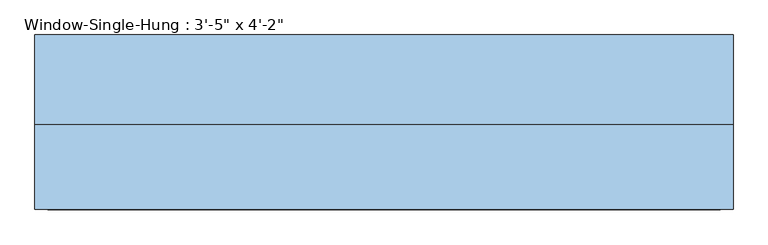
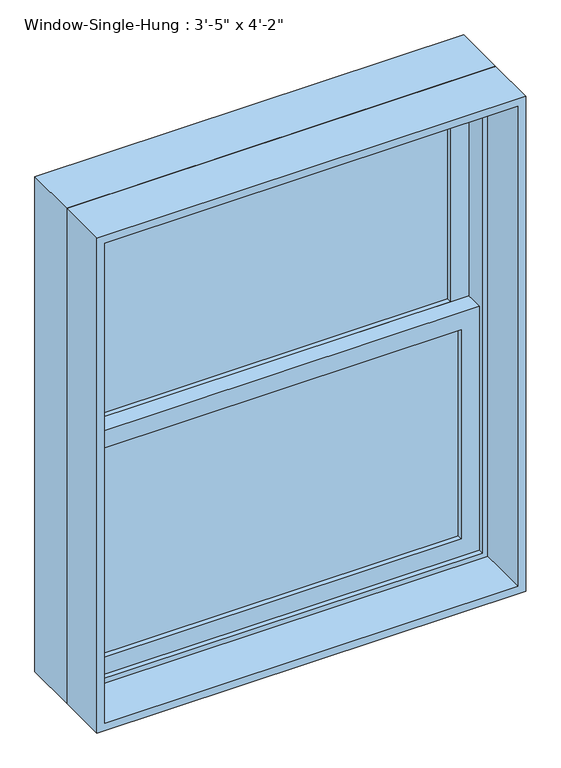
"""IFC4 building model written with IfcOpenShell, lengths in millimetres: window geometry."""

import ifcopenshell
import ifcopenshell.guid

model = None  # the IFC model being written
_history = None  # IfcOwnerHistory: only IFC2X3 demands one
_inside = {}  # id of a spatial element -> (the spatial element, [elements in it])
_under = {}  # id of a project, library or spatial element -> (it, [spatial elements below it])
_declared = {}  # id of a project -> (the project, [libraries it declares])
_typed = {}  # id of a type object -> (the type object, [elements of that type])
_made_of = {}  # id of a material, layer set ... -> (it, [elements and type objects made of it])


def new_model(schema):
    """Start an empty IFC model of exactly this schema.

    Asked for "IFC4X3", IfcOpenShell would pick the latest addendum, in which some entities
    have other attributes; the version numbers below select the first issue.
    IFC2X3 requires an IfcOwnerHistory on every rooted entity: one is made here for all.
    """
    global model, _history
    if schema == "IFC4X3":
        model = ifcopenshell.file(schema_version=(4, 3, 0, 0))
    else:
        model = ifcopenshell.file(schema=schema)
    _inside.clear()
    _under.clear()
    _declared.clear()
    _typed.clear()
    _made_of.clear()
    _history = None
    if model.schema == "IFC2X3":
        org = make("IfcOrganization", Name="unknown")
        user = make(
            "IfcPersonAndOrganization",
            ThePerson=make("IfcPerson", FamilyName="unknown"),
            TheOrganization=org,
        )
        app = make(
            "IfcApplication",
            ApplicationDeveloper=org,
            Version="unknown",
            ApplicationFullName="unknown",
            ApplicationIdentifier="unknown",
        )
        _history = make(
            "IfcOwnerHistory",
            OwningUser=user,
            OwningApplication=app,
            ChangeAction="ADDED",
            CreationDate=0,
        )
    return model


def make(cls, **values):
    """One entity of the class cls with the attributes given. An attribute that is None is left unset."""
    return model.create_entity(
        cls, **{name: value for name, value in values.items() if value is not None}
    )


def rooted(cls, **values):
    """An entity with a GlobalId (a new one), such as an element, a storey or a relation."""
    return make(cls, GlobalId=ifcopenshell.guid.new(), OwnerHistory=_history, **values)


def si_unit(unit_type, name, prefix=None):
    """IfcSIUnit, for example si_unit("LENGTHUNIT", "METRE", prefix="MILLI")."""
    return make("IfcSIUnit", UnitType=unit_type, Prefix=prefix, Name=name)


def assignment(units):
    """IfcUnitAssignment: the units of a project."""
    return None if units is None else make("IfcUnitAssignment", Units=units)


def point(xyz):
    """IfcCartesianPoint."""
    return None if xyz is None else make("IfcCartesianPoint", Coordinates=xyz)


def direction(xyz):
    """IfcDirection."""
    return None if xyz is None else make("IfcDirection", DirectionRatios=xyz)


def frame(location, z_axis=None, x_axis=None):
    """IfcAxis2Placement3D, a coordinate frame: its origin and axes. An axis left out is left unset."""
    return make(
        "IfcAxis2Placement3D",
        Location=point(location),
        Axis=direction(z_axis),
        RefDirection=direction(x_axis),
    )


def origin():
    """The frame at (0, 0, 0) with its axes left unset."""
    return frame((0.0, 0.0, 0.0))


def place(relative_to, where):
    """IfcLocalPlacement: puts the frame where relative to a parent placement (None: the world)."""
    return make(
        "IfcLocalPlacement", PlacementRelTo=relative_to, RelativePlacement=where
    )


def context(
    kind, dimensions, precision=None, world=None, true_north=None, identifier=None
):
    """IfcGeometricRepresentationContext, for example the 3D "Model" context."""
    return make(
        "IfcGeometricRepresentationContext",
        ContextIdentifier=identifier,
        ContextType=kind,
        CoordinateSpaceDimension=dimensions,
        Precision=precision,
        WorldCoordinateSystem=world,
        TrueNorth=true_north,
    )


def project(units=None, contexts=None):
    """IfcProject with its units and contexts."""
    return rooted(
        "IfcProject",
        Name="project",
        RepresentationContexts=contexts,
        UnitsInContext=assignment(units),
    )


def spatial(cls, under=None, at=None, **own):
    """A site, building, storey or space (cls), placed at a placement, below another one or the project."""
    s = rooted(cls, ObjectPlacement=at, **own)
    if under is not None:
        _under.setdefault(under.id(), (under, []))[1].append(s)
    return s


def polyline(points):
    """IfcPolyline through the points."""
    return make("IfcPolyline", Points=[point(p) for p in points])


def outline(outer, holes=None, kind="AREA"):
    """IfcArbitraryClosedProfileDef: a profile drawn as a closed curve; with holes, ...WithVoids."""
    if holes is None:
        return make("IfcArbitraryClosedProfileDef", ProfileType=kind, OuterCurve=outer)
    return make(
        "IfcArbitraryProfileDefWithVoids",
        ProfileType=kind,
        OuterCurve=outer,
        InnerCurves=holes,
    )


def extrude(swept, where, along, depth):
    """IfcExtrudedAreaSolid: the profile swept, set in the frame where, extruded along a direction by depth."""
    return make(
        "IfcExtrudedAreaSolid",
        SweptArea=swept,
        Position=where,
        ExtrudedDirection=direction(along),
        Depth=depth,
    )


def shape(context_of_items, identifier, shape_type, items):
    """IfcShapeRepresentation: the items that make up one representation, for example the "Body"."""
    return make(
        "IfcShapeRepresentation",
        ContextOfItems=context_of_items,
        RepresentationIdentifier=identifier,
        RepresentationType=shape_type,
        Items=items,
    )


def source(mapping_origin, context_of_items, identifier, shape_type, items):
    """IfcRepresentationMap: a shape defined once, which mapped items show again and again."""
    return make(
        "IfcRepresentationMap",
        MappingOrigin=mapping_origin,
        MappedRepresentation=shape(context_of_items, identifier, shape_type, items),
    )


def transform(
    local_origin,
    x_axis=None,
    y_axis=None,
    z_axis=None,
    scale=None,
    scale2=None,
    scale3=None,
    uniform=True,
):
    """IfcCartesianTransformationOperator3D, or its non-uniform kind. x_axis, y_axis, z_axis: its Axis1, 2, 3."""
    if uniform:
        return make(
            "IfcCartesianTransformationOperator3D",
            Axis1=direction(x_axis),
            Axis2=direction(y_axis),
            LocalOrigin=point(local_origin),
            Scale=scale,
            Axis3=direction(z_axis),
        )
    return make(
        "IfcCartesianTransformationOperator3DnonUniform",
        Axis1=direction(x_axis),
        Axis2=direction(y_axis),
        LocalOrigin=point(local_origin),
        Scale=scale,
        Axis3=direction(z_axis),
        Scale2=scale2,
        Scale3=scale3,
    )


def mapped(mapping_source, mapping_target):
    """IfcMappedItem: shows the shape of a source again, moved by a transform."""
    return make(
        "IfcMappedItem", MappingSource=mapping_source, MappingTarget=mapping_target
    )


def made_of(thing, what):
    """Note that an element or type object is made of a material, layer set ...; save() writes the relation."""
    if what is not None:
        _made_of.setdefault(what.id(), (what, []))[1].append(thing)
    return thing


def element(
    cls,
    number,
    at=None,
    inside=None,
    cuts=None,
    type_object=None,
    material=None,
    context=None,
    identifier="Body",
    shape_type=None,
    held_by="IfcProductDefinitionShape",
    body=None,
    shapes=None,
    **own,
):
    """One element of the class cls, such as IfcWall. Its Tag is "e" and its number.

    at: its placement. inside: the storey or other place that contains it. cuts: it is an
    opening in that element (IfcRelVoidsElement). A single representation is given by context,
    identifier, shape_type and body (its items); several are given by shapes. held_by: the class
    of the entity that holds the representations. save() writes the other relations.
    """
    e = rooted(cls, Tag="e%d" % number, ObjectPlacement=at, **own)
    if body is not None:
        shapes = [shape(context, identifier, shape_type, body)]
    if shapes is not None:
        e.Representation = make(held_by, Representations=shapes)
    if inside is not None:
        _inside.setdefault(inside.id(), (inside, []))[1].append(e)
    if cuts is not None:
        rooted(
            "IfcRelVoidsElement", RelatingBuildingElement=cuts, RelatedOpeningElement=e
        )
    if type_object is not None:
        _typed.setdefault(type_object.id(), (type_object, []))[1].append(e)
    return made_of(e, material)


def aggregate(whole, parts):
    """IfcRelAggregates: a whole, such as a stair, and the parts it consists of."""
    return rooted("IfcRelAggregates", RelatingObject=whole, RelatedObjects=parts)


def save(model, path):
    """Write the relations noted so far, then the file.

    IfcRelAggregates (storeys below a building ...), IfcRelContainedInSpatialStructure (elements
    in a storey), IfcRelDefinesByType, IfcRelAssociatesMaterial and IfcRelDeclares: one each for
    every whole, place, type object, material and project.
    """
    for whole, parts in _under.values():
        aggregate(whole, parts)
    for where, things in _inside.values():
        rooted(
            "IfcRelContainedInSpatialStructure",
            RelatedElements=things,
            RelatingStructure=where,
        )
    for kind, things in _typed.values():
        rooted("IfcRelDefinesByType", RelatedObjects=things, RelatingType=kind)
    for what, things in _made_of.values():
        rooted("IfcRelAssociatesMaterial", RelatedObjects=things, RelatingMaterial=what)
    for by, libraries in _declared.values():
        rooted("IfcRelDeclares", RelatingContext=by, RelatedDefinitions=libraries)
    model.write(path)


def window_7112179c(model_context):
    return source(origin(), model_context, "Body", "SweptSolid", [
        extrude(outline(polyline([(444.5, 50.8), (444.5, 44.45), (-444.5, 44.45), (-444.5, 50.8), (444.5, 50.8)])), frame((0.0, 0.0, 990.6), z_axis=(0.0, 0.0, 1.0), x_axis=(1.0, 0.0, 0.0)), (0.0, 0.0, 1.0), 536.575),
        extrude(outline(polyline([(-444.5, 38.1), (444.5, 38.1), (444.5, 31.75), (-444.5, 31.75), (-444.5, 38.1)])), frame((0.0, 0.0, 990.6), z_axis=(0.0, 0.0, 1.0), x_axis=(1.0, 0.0, 0.0)), (0.0, 0.0, 1.0), 536.575),
        extrude(outline(polyline([(444.5, 95.25), (444.5, 88.9), (-444.5, 88.9), (-444.5, 95.25), (444.5, 95.25)])), frame((0.0, 0.0, 1571.625), z_axis=(0.0, 0.0, 1.0), x_axis=(1.0, 0.0, 0.0)), (0.0, 0.0, 1.0), 536.575),
        extrude(outline(polyline([(-444.5, 82.55), (444.5, 82.55), (444.5, 76.2), (-444.5, 76.2), (-444.5, 82.55)])), frame((0.0, 0.0, 1571.625), z_axis=(0.0, 0.0, 1.0), x_axis=(1.0, 0.0, 0.0)), (0.0, 0.0, 1.0), 536.575),
        extrude(outline(polyline([(1571.625, -488.95), (946.15, -488.95), (946.15, 488.95), (1571.625, 488.95), (1571.625, -488.95)]), holes=[polyline([(1527.175, 444.5), (990.6, 444.5), (990.6, -444.5), (1527.175, -444.5), (1527.175, 444.5)])]), frame((0.0, 19.05, 0.0), z_axis=(0.0, 1.0, 0.0), x_axis=(0.0, 0.0, 1.0)), (0.0, 0.0, 1.0), 44.45),
        extrude(outline(polyline([(2152.65, -488.95), (1527.175, -488.95), (1527.175, 488.95), (2152.65, 488.95), (2152.65, -488.95)]), holes=[polyline([(2108.2, 444.5), (1571.625, 444.5), (1571.625, -444.5), (2108.2, -444.5), (2108.2, 444.5)])]), frame((0.0, 63.5, 0.0), z_axis=(0.0, 1.0, 0.0), x_axis=(0.0, 0.0, 1.0)), (0.0, 0.0, 1.0), 44.45),
        extrude(outline(polyline([(2184.4, -520.7), (914.4, -520.7), (914.4, 520.7), (2184.4, 520.7), (2184.4, -520.7)]), holes=[polyline([(2152.65, 488.95), (946.15, 488.95), (946.15, -488.95), (2152.65, -488.95), (2152.65, 488.95)])]), frame((0.0, 6.35, 0.0), z_axis=(0.0, 1.0, 0.0), x_axis=(0.0, 0.0, 1.0)), (0.0, 0.0, 1.0), 133.35),
        extrude(outline(polyline([(2184.4, 520.7), (2184.4, -520.7), (914.4, -520.7), (914.4, 520.7), (2184.4, 520.7)]), holes=[polyline([(2165.35, 501.65), (933.45, 501.65), (933.45, -501.65), (2165.35, -501.65), (2165.35, 501.65)])]), frame((0.0, -120.65, 0.0), z_axis=(0.0, 1.0, 0.0), x_axis=(0.0, 0.0, 1.0)), (0.0, 0.0, 1.0), 127.0),
    ])


if __name__ == "__main__":
    model = new_model("IFC4")
    model_context = context("Model", 3, world=origin())
    ifc_project = project(units=[si_unit("LENGTHUNIT", "METRE", prefix="MILLI")], contexts=[model_context])
    site = spatial("IfcSite", under=ifc_project)
    building = spatial("IfcBuilding", under=site)
    placement = place(None, origin())
    window_shape = window_7112179c(model_context)
    element("IfcWindow", 1, ObjectType="Window-Single-Hung : 3'-5\" x 4'-2\"", at=placement, inside=building, context=model_context, shape_type="MappedRepresentation", body=[
        mapped(window_shape, transform((0.0, 0.0, 0.0), x_axis=(1.0, 0.0, 0.0), y_axis=(0.0, 1.0, 0.0), z_axis=(0.0, 0.0, 1.0))),
    ])
    save(model, "model.ifc")

# Revit data of these elements
# Type "Window-Single-Hung : 3'-5\" x 4'-2\""
#   Type Mark = "24"
#   Fire Rating = "0.5h"
#   Construction Type Id = "DG-DR"
#   Assembly Code = "B2020100"
#   Analytic Construction = "Double glazing - domestic"
#   Wall Thickness [instance default] = 0' - 6"
#   Window Inset [instance default] = 0' - 0"
#   Visual Light Transmittance = 0.81
#   Thermal Resistance (R) = 0.319569 (m²·K)/W
#   Solar Heat Gain Coefficient = 0.76
#   Muntin Width = 2' - 11"
#   Muntin Height = 1' - 9 1/8"
#   Interior Wall Closure [instance default] = 0' - 1 1/2"
#   Rough Width = 3' - 5 1/2"
#   Rough Height = 4' - 2 1/2"
#   Frame Extension [instance default] = 0' - 1 1/4"
#   Exterior Wall Closure [instance default] = 0' - 0 1/2"
#   Extension Jamb [instance default] = 0' - 1 1/2"
#   Heat Transfer Coefficient (U) = 3.12929 W/(m²·K)
#   Height = 4' - 2"
#   Width = 3' - 5"
#   Top Muntin Visibility = no
#   Indicator Visibility = no
#   Extension Jamb Visibility [instance default] = yes
#   Interior Trim Visibility [instance default] = yes
#   Exterior Trim Visibility [instance default] = yes
#   Bottom Muntin Visibility = no
#   Muntin Pattern = Muntin Pattern_2x2 : Muntin Pattern_2x2
#   Interior Trim Material = Wood - Stained
#   Interior Trim = Trim-Window-Interior-Flat : Picture Frame
#   Exterior Trim Material = Clad - White
#   Exterior Trim = Trim-Window-Exterior-Flat : with Sill
#   Glass Panel Material = Glass
#   Exterior Frame Material = Clad - White
#   Interior Frame Material = Wood - Stained
#   Wall Closure = (empty or 0)
# Element 1 (IfcWindow, "Window-Single-Hung : 3'-5\" x 4'-2\"")
#   Wall Thickness = 0' - 9 1/2"
#   Extension Jamb = 0' - 5"
#   Materials on its faces: "Wood - Stained", "Glass", "Clad - White"
# Materials
#   "Wood - Stained": class "Wood", colour RGB 224 178 126, transparency 0, Cost = 0
#   "Clad - White": class "Wood", colour RGB 242 242 238, transparency 0, Cost = 0
#   "Glass": class "Glass", colour RGB 218 227 224, transparency 0.85, Description = "Soda Lime Glass", Cost = 0
